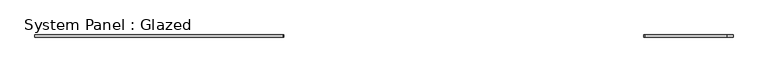
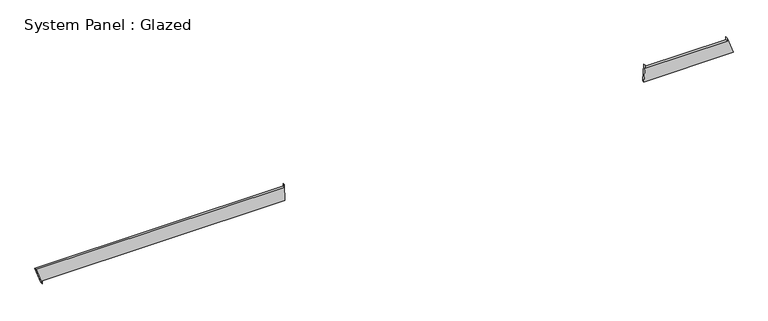
"""IFC4 building model written with IfcOpenShell, lengths in millimetres: plate geometry, System Panel : Glazed."""

import ifcopenshell
import ifcopenshell.guid

model = None  # the IFC model being written
_history = None  # IfcOwnerHistory: only IFC2X3 demands one
_inside = {}  # id of a spatial element -> (the spatial element, [elements in it])
_under = {}  # id of a project, library or spatial element -> (it, [spatial elements below it])
_declared = {}  # id of a project -> (the project, [libraries it declares])
_typed = {}  # id of a type object -> (the type object, [elements of that type])
_made_of = {}  # id of a material, layer set ... -> (it, [elements and type objects made of it])


def new_model(schema):
    """Start an empty IFC model of exactly this schema.

    Asked for "IFC4X3", IfcOpenShell would pick the latest addendum, in which some entities
    have other attributes; the version numbers below select the first issue.
    IFC2X3 requires an IfcOwnerHistory on every rooted entity: one is made here for all.
    """
    global model, _history
    if schema == "IFC4X3":
        model = ifcopenshell.file(schema_version=(4, 3, 0, 0))
    else:
        model = ifcopenshell.file(schema=schema)
    _inside.clear()
    _under.clear()
    _declared.clear()
    _typed.clear()
    _made_of.clear()
    _history = None
    if model.schema == "IFC2X3":
        org = make("IfcOrganization", Name="unknown")
        user = make(
            "IfcPersonAndOrganization",
            ThePerson=make("IfcPerson", FamilyName="unknown"),
            TheOrganization=org,
        )
        app = make(
            "IfcApplication",
            ApplicationDeveloper=org,
            Version="unknown",
            ApplicationFullName="unknown",
            ApplicationIdentifier="unknown",
        )
        _history = make(
            "IfcOwnerHistory",
            OwningUser=user,
            OwningApplication=app,
            ChangeAction="ADDED",
            CreationDate=0,
        )
    return model


def make(cls, **values):
    """One entity of the class cls with the attributes given. An attribute that is None is left unset."""
    return model.create_entity(
        cls, **{name: value for name, value in values.items() if value is not None}
    )


def rooted(cls, **values):
    """An entity with a GlobalId (a new one), such as an element, a storey or a relation."""
    return make(cls, GlobalId=ifcopenshell.guid.new(), OwnerHistory=_history, **values)


def si_unit(unit_type, name, prefix=None):
    """IfcSIUnit, for example si_unit("LENGTHUNIT", "METRE", prefix="MILLI")."""
    return make("IfcSIUnit", UnitType=unit_type, Prefix=prefix, Name=name)


def assignment(units):
    """IfcUnitAssignment: the units of a project."""
    return None if units is None else make("IfcUnitAssignment", Units=units)


def point(xyz):
    """IfcCartesianPoint."""
    return None if xyz is None else make("IfcCartesianPoint", Coordinates=xyz)


def direction(xyz):
    """IfcDirection."""
    return None if xyz is None else make("IfcDirection", DirectionRatios=xyz)


def frame(location, z_axis=None, x_axis=None):
    """IfcAxis2Placement3D, a coordinate frame: its origin and axes. An axis left out is left unset."""
    return make(
        "IfcAxis2Placement3D",
        Location=point(location),
        Axis=direction(z_axis),
        RefDirection=direction(x_axis),
    )


def origin():
    """The frame at (0, 0, 0) with its axes left unset."""
    return frame((0.0, 0.0, 0.0))


def place(relative_to, where):
    """IfcLocalPlacement: puts the frame where relative to a parent placement (None: the world)."""
    return make(
        "IfcLocalPlacement", PlacementRelTo=relative_to, RelativePlacement=where
    )


def context(
    kind, dimensions, precision=None, world=None, true_north=None, identifier=None
):
    """IfcGeometricRepresentationContext, for example the 3D "Model" context."""
    return make(
        "IfcGeometricRepresentationContext",
        ContextIdentifier=identifier,
        ContextType=kind,
        CoordinateSpaceDimension=dimensions,
        Precision=precision,
        WorldCoordinateSystem=world,
        TrueNorth=true_north,
    )


def project(units=None, contexts=None):
    """IfcProject with its units and contexts."""
    return rooted(
        "IfcProject",
        Name="project",
        RepresentationContexts=contexts,
        UnitsInContext=assignment(units),
    )


def spatial(cls, under=None, at=None, **own):
    """A site, building, storey or space (cls), placed at a placement, below another one or the project."""
    s = rooted(cls, ObjectPlacement=at, **own)
    if under is not None:
        _under.setdefault(under.id(), (under, []))[1].append(s)
    return s


def polyline(points):
    """IfcPolyline through the points."""
    return make("IfcPolyline", Points=[point(p) for p in points])


def outline(outer, holes=None, kind="AREA"):
    """IfcArbitraryClosedProfileDef: a profile drawn as a closed curve; with holes, ...WithVoids."""
    if holes is None:
        return make("IfcArbitraryClosedProfileDef", ProfileType=kind, OuterCurve=outer)
    return make(
        "IfcArbitraryProfileDefWithVoids",
        ProfileType=kind,
        OuterCurve=outer,
        InnerCurves=holes,
    )


def extrude(swept, where, along, depth):
    """IfcExtrudedAreaSolid: the profile swept, set in the frame where, extruded along a direction by depth."""
    return make(
        "IfcExtrudedAreaSolid",
        SweptArea=swept,
        Position=where,
        ExtrudedDirection=direction(along),
        Depth=depth,
    )


def shape(context_of_items, identifier, shape_type, items):
    """IfcShapeRepresentation: the items that make up one representation, for example the "Body"."""
    return make(
        "IfcShapeRepresentation",
        ContextOfItems=context_of_items,
        RepresentationIdentifier=identifier,
        RepresentationType=shape_type,
        Items=items,
    )


def source(mapping_origin, context_of_items, identifier, shape_type, items):
    """IfcRepresentationMap: a shape defined once, which mapped items show again and again."""
    return make(
        "IfcRepresentationMap",
        MappingOrigin=mapping_origin,
        MappedRepresentation=shape(context_of_items, identifier, shape_type, items),
    )


def transform(
    local_origin,
    x_axis=None,
    y_axis=None,
    z_axis=None,
    scale=None,
    scale2=None,
    scale3=None,
    uniform=True,
):
    """IfcCartesianTransformationOperator3D, or its non-uniform kind. x_axis, y_axis, z_axis: its Axis1, 2, 3."""
    if uniform:
        return make(
            "IfcCartesianTransformationOperator3D",
            Axis1=direction(x_axis),
            Axis2=direction(y_axis),
            LocalOrigin=point(local_origin),
            Scale=scale,
            Axis3=direction(z_axis),
        )
    return make(
        "IfcCartesianTransformationOperator3DnonUniform",
        Axis1=direction(x_axis),
        Axis2=direction(y_axis),
        LocalOrigin=point(local_origin),
        Scale=scale,
        Axis3=direction(z_axis),
        Scale2=scale2,
        Scale3=scale3,
    )


def mapped(mapping_source, mapping_target):
    """IfcMappedItem: shows the shape of a source again, moved by a transform."""
    return make(
        "IfcMappedItem", MappingSource=mapping_source, MappingTarget=mapping_target
    )


def made_of(thing, what):
    """Note that an element or type object is made of a material, layer set ...; save() writes the relation."""
    if what is not None:
        _made_of.setdefault(what.id(), (what, []))[1].append(thing)
    return thing


def element(
    cls,
    number,
    at=None,
    inside=None,
    cuts=None,
    type_object=None,
    material=None,
    context=None,
    identifier="Body",
    shape_type=None,
    held_by="IfcProductDefinitionShape",
    body=None,
    shapes=None,
    **own,
):
    """One element of the class cls, such as IfcWall. Its Tag is "e" and its number.

    at: its placement. inside: the storey or other place that contains it. cuts: it is an
    opening in that element (IfcRelVoidsElement). A single representation is given by context,
    identifier, shape_type and body (its items); several are given by shapes. held_by: the class
    of the entity that holds the representations. save() writes the other relations.
    """
    e = rooted(cls, Tag="e%d" % number, ObjectPlacement=at, **own)
    if body is not None:
        shapes = [shape(context, identifier, shape_type, body)]
    if shapes is not None:
        e.Representation = make(held_by, Representations=shapes)
    if inside is not None:
        _inside.setdefault(inside.id(), (inside, []))[1].append(e)
    if cuts is not None:
        rooted(
            "IfcRelVoidsElement", RelatingBuildingElement=cuts, RelatedOpeningElement=e
        )
    if type_object is not None:
        _typed.setdefault(type_object.id(), (type_object, []))[1].append(e)
    return made_of(e, material)


def aggregate(whole, parts):
    """IfcRelAggregates: a whole, such as a stair, and the parts it consists of."""
    return rooted("IfcRelAggregates", RelatingObject=whole, RelatedObjects=parts)


def save(model, path):
    """Write the relations noted so far, then the file.

    IfcRelAggregates (storeys below a building ...), IfcRelContainedInSpatialStructure (elements
    in a storey), IfcRelDefinesByType, IfcRelAssociatesMaterial and IfcRelDeclares: one each for
    every whole, place, type object, material and project.
    """
    for whole, parts in _under.values():
        aggregate(whole, parts)
    for where, things in _inside.values():
        rooted(
            "IfcRelContainedInSpatialStructure",
            RelatedElements=things,
            RelatingStructure=where,
        )
    for kind, things in _typed.values():
        rooted("IfcRelDefinesByType", RelatedObjects=things, RelatingType=kind)
    for what, things in _made_of.values():
        rooted("IfcRelAssociatesMaterial", RelatedObjects=things, RelatingMaterial=what)
    for by, libraries in _declared.values():
        rooted("IfcRelDeclares", RelatingContext=by, RelatedDefinitions=libraries)
    model.write(path)


def system_panel_glazed_6db51844(model_context):
    return source(origin(), model_context, "Body", "SweptSolid", [
        extrude(outline(polyline([(0.0, -3959.2274782), (35.3553391, -3959.2274782), (35.3553391, -1154.1262772), (234.7828866, -1159.7546078), (199.4275476, -1159.7542894), (199.4017187, -4027.8928943), (0.0, -3959.2274782)])), frame((0.0, -49.5, 0.0), z_axis=(0.0, 1.0, 0.0), x_axis=(0.0, 0.0, 1.0)), (0.0, 0.0, 1.0), 25.0),
        extrude(outline(polyline([(35.3553391, 2996.1724344), (35.3553391, 4027.8928943), (234.8289868, 3959.4017402), (199.4736478, 3959.4020585), (199.4651053, 3010.8153043), (234.8204444, 3010.814986), (35.3553391, 2996.1724344)])), frame((0.0, -49.5, 0.0), z_axis=(0.0, 1.0, 0.0), x_axis=(0.0, 0.0, 1.0)), (0.0, 0.0, 1.0), 25.0),
    ])


if __name__ == "__main__":
    model = new_model("IFC4")
    model_context = context("Model", 3, world=origin())
    ifc_project = project(units=[si_unit("LENGTHUNIT", "METRE", prefix="MILLI")], contexts=[model_context])
    site = spatial("IfcSite", under=ifc_project)
    building = spatial("IfcBuilding", under=site)
    placement = place(None, origin())
    system_panel_glazed_shape = system_panel_glazed_6db51844(model_context)
    element("IfcPlate", 1, ObjectType="System Panel : Glazed", at=placement, inside=building, context=model_context, shape_type="MappedRepresentation", body=[
        mapped(system_panel_glazed_shape, transform((0.0, 0.0, 0.0), x_axis=(1.0, 0.0, 0.0), y_axis=(0.0, 1.0, 0.0), z_axis=(0.0, 0.0, 1.0))),
    ])
    save(model, "model.ifc")

# Revit data of these elements
# Element 1 (IfcPlate, "System Panel : Glazed")
#   Materials on its faces: "Glass"
# Materials
#   "Glass": class "Glass", colour RGB 218 227 224, transparency 0.85, Description = "Soda Lime Glass", Cost = 0
